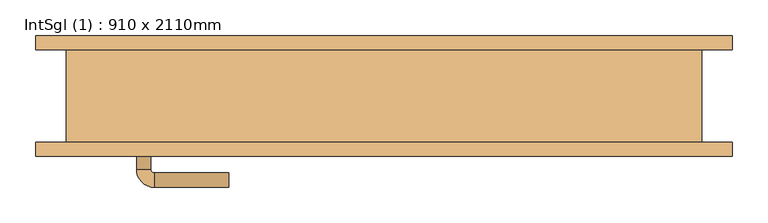
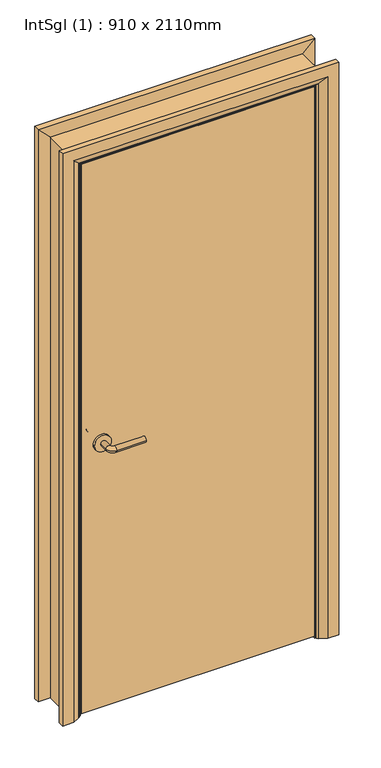
"""IFC4 building model written with IfcOpenShell, lengths in millimetres: door geometry, IntSgl (1) : 910 x 2110mm."""

import ifcopenshell
import ifcopenshell.guid

model = None  # the IFC model being written
_history = None  # IfcOwnerHistory: only IFC2X3 demands one
_inside = {}  # id of a spatial element -> (the spatial element, [elements in it])
_under = {}  # id of a project, library or spatial element -> (it, [spatial elements below it])
_declared = {}  # id of a project -> (the project, [libraries it declares])
_typed = {}  # id of a type object -> (the type object, [elements of that type])
_made_of = {}  # id of a material, layer set ... -> (it, [elements and type objects made of it])


def new_model(schema):
    """Start an empty IFC model of exactly this schema.

    Asked for "IFC4X3", IfcOpenShell would pick the latest addendum, in which some entities
    have other attributes; the version numbers below select the first issue.
    IFC2X3 requires an IfcOwnerHistory on every rooted entity: one is made here for all.
    """
    global model, _history
    if schema == "IFC4X3":
        model = ifcopenshell.file(schema_version=(4, 3, 0, 0))
    else:
        model = ifcopenshell.file(schema=schema)
    _inside.clear()
    _under.clear()
    _declared.clear()
    _typed.clear()
    _made_of.clear()
    _history = None
    if model.schema == "IFC2X3":
        org = make("IfcOrganization", Name="unknown")
        user = make(
            "IfcPersonAndOrganization",
            ThePerson=make("IfcPerson", FamilyName="unknown"),
            TheOrganization=org,
        )
        app = make(
            "IfcApplication",
            ApplicationDeveloper=org,
            Version="unknown",
            ApplicationFullName="unknown",
            ApplicationIdentifier="unknown",
        )
        _history = make(
            "IfcOwnerHistory",
            OwningUser=user,
            OwningApplication=app,
            ChangeAction="ADDED",
            CreationDate=0,
        )
    return model


def make(cls, **values):
    """One entity of the class cls with the attributes given. An attribute that is None is left unset."""
    return model.create_entity(
        cls, **{name: value for name, value in values.items() if value is not None}
    )


def rooted(cls, **values):
    """An entity with a GlobalId (a new one), such as an element, a storey or a relation."""
    return make(cls, GlobalId=ifcopenshell.guid.new(), OwnerHistory=_history, **values)


def si_unit(unit_type, name, prefix=None):
    """IfcSIUnit, for example si_unit("LENGTHUNIT", "METRE", prefix="MILLI")."""
    return make("IfcSIUnit", UnitType=unit_type, Prefix=prefix, Name=name)


def assignment(units):
    """IfcUnitAssignment: the units of a project."""
    return None if units is None else make("IfcUnitAssignment", Units=units)


def point(xyz):
    """IfcCartesianPoint."""
    return None if xyz is None else make("IfcCartesianPoint", Coordinates=xyz)


def direction(xyz):
    """IfcDirection."""
    return None if xyz is None else make("IfcDirection", DirectionRatios=xyz)


def frame(location, z_axis=None, x_axis=None):
    """IfcAxis2Placement3D, a coordinate frame: its origin and axes. An axis left out is left unset."""
    return make(
        "IfcAxis2Placement3D",
        Location=point(location),
        Axis=direction(z_axis),
        RefDirection=direction(x_axis),
    )


def frame_2d(location, x_axis=None):
    """IfcAxis2Placement2D, a coordinate frame in the plane: its origin and x axis."""
    return make(
        "IfcAxis2Placement2D", Location=point(location), RefDirection=direction(x_axis)
    )


def origin():
    """The frame at (0, 0, 0) with its axes left unset."""
    return frame((0.0, 0.0, 0.0))


def place(relative_to, where):
    """IfcLocalPlacement: puts the frame where relative to a parent placement (None: the world)."""
    return make(
        "IfcLocalPlacement", PlacementRelTo=relative_to, RelativePlacement=where
    )


def context(
    kind, dimensions, precision=None, world=None, true_north=None, identifier=None
):
    """IfcGeometricRepresentationContext, for example the 3D "Model" context."""
    return make(
        "IfcGeometricRepresentationContext",
        ContextIdentifier=identifier,
        ContextType=kind,
        CoordinateSpaceDimension=dimensions,
        Precision=precision,
        WorldCoordinateSystem=world,
        TrueNorth=true_north,
    )


def project(units=None, contexts=None):
    """IfcProject with its units and contexts."""
    return rooted(
        "IfcProject",
        Name="project",
        RepresentationContexts=contexts,
        UnitsInContext=assignment(units),
    )


def spatial(cls, under=None, at=None, **own):
    """A site, building, storey or space (cls), placed at a placement, below another one or the project."""
    s = rooted(cls, ObjectPlacement=at, **own)
    if under is not None:
        _under.setdefault(under.id(), (under, []))[1].append(s)
    return s


def polyline(points):
    """IfcPolyline through the points."""
    return make("IfcPolyline", Points=[point(p) for p in points])


def circle_curve(where, radius):
    """IfcCircle in the frame where."""
    return make("IfcCircle", Position=where, Radius=radius)


def ellipse_curve(where, semi_axis1, semi_axis2):
    """IfcEllipse in the frame where."""
    return make(
        "IfcEllipse", Position=where, SemiAxis1=semi_axis1, SemiAxis2=semi_axis2
    )


def trimmed(basis, trim1, trim2, sense, master):
    """IfcTrimmedCurve: the piece of a basis curve between two trims."""
    return make(
        "IfcTrimmedCurve",
        BasisCurve=basis,
        Trim1=trim1,
        Trim2=trim2,
        SenseAgreement=sense,
        MasterRepresentation=master,
    )


def segment(curve, same_sense, transition):
    """IfcCompositeCurveSegment."""
    return make(
        "IfcCompositeCurveSegment",
        Transition=transition,
        SameSense=same_sense,
        ParentCurve=curve,
    )


def composite_curve(segments, self_intersect=None):
    """IfcCompositeCurve: segments joined end to end."""
    return make("IfcCompositeCurve", Segments=segments, SelfIntersect=self_intersect)


def outline(outer, holes=None, kind="AREA"):
    """IfcArbitraryClosedProfileDef: a profile drawn as a closed curve; with holes, ...WithVoids."""
    if holes is None:
        return make("IfcArbitraryClosedProfileDef", ProfileType=kind, OuterCurve=outer)
    return make(
        "IfcArbitraryProfileDefWithVoids",
        ProfileType=kind,
        OuterCurve=outer,
        InnerCurves=holes,
    )


def extrude(swept, where, along, depth):
    """IfcExtrudedAreaSolid: the profile swept, set in the frame where, extruded along a direction by depth."""
    return make(
        "IfcExtrudedAreaSolid",
        SweptArea=swept,
        Position=where,
        ExtrudedDirection=direction(along),
        Depth=depth,
    )


def faces_of(points, faces, orient=None, outer=None):
    """IfcFace entities. A face is a list of loops; a loop is a list of indices into points, from 0.

    orient and outer hold one flag for each loop. By default every Orientation is true, the
    first loop of a face is its IfcFaceOuterBound and the others are IfcFaceBound.
    """
    made = []
    for i, loops in enumerate(faces):
        bounds = []
        for j, loop in enumerate(loops):
            is_outer = j == 0 if outer is None else outer[i][j]
            bounds.append(
                make(
                    "IfcFaceOuterBound" if is_outer else "IfcFaceBound",
                    Bound=make("IfcPolyLoop", Polygon=[points[k] for k in loop]),
                    Orientation=True if orient is None else orient[i][j],
                )
            )
        made.append(make("IfcFace", Bounds=bounds))
    return made


def faceted_brep(points, faces, orient=None, outer=None, voids=None):
    """IfcFacetedBrep: a solid bounded by flat faces; with voids (closed shells), ...WithVoids."""
    shared = [point(p) for p in points]
    hull = make("IfcClosedShell", CfsFaces=faces_of(shared, faces, orient, outer))
    if voids is None:
        return make("IfcFacetedBrep", Outer=hull)
    return make(
        "IfcFacetedBrepWithVoids",
        Outer=hull,
        Voids=[
            make(cls, CfsFaces=faces_of(shared, fs, o, b)) for cls, fs, o, b in voids
        ],
    )


def shape(context_of_items, identifier, shape_type, items):
    """IfcShapeRepresentation: the items that make up one representation, for example the "Body"."""
    return make(
        "IfcShapeRepresentation",
        ContextOfItems=context_of_items,
        RepresentationIdentifier=identifier,
        RepresentationType=shape_type,
        Items=items,
    )


def source(mapping_origin, context_of_items, identifier, shape_type, items):
    """IfcRepresentationMap: a shape defined once, which mapped items show again and again."""
    return make(
        "IfcRepresentationMap",
        MappingOrigin=mapping_origin,
        MappedRepresentation=shape(context_of_items, identifier, shape_type, items),
    )


def transform(
    local_origin,
    x_axis=None,
    y_axis=None,
    z_axis=None,
    scale=None,
    scale2=None,
    scale3=None,
    uniform=True,
):
    """IfcCartesianTransformationOperator3D, or its non-uniform kind. x_axis, y_axis, z_axis: its Axis1, 2, 3."""
    if uniform:
        return make(
            "IfcCartesianTransformationOperator3D",
            Axis1=direction(x_axis),
            Axis2=direction(y_axis),
            LocalOrigin=point(local_origin),
            Scale=scale,
            Axis3=direction(z_axis),
        )
    return make(
        "IfcCartesianTransformationOperator3DnonUniform",
        Axis1=direction(x_axis),
        Axis2=direction(y_axis),
        LocalOrigin=point(local_origin),
        Scale=scale,
        Axis3=direction(z_axis),
        Scale2=scale2,
        Scale3=scale3,
    )


def mapped(mapping_source, mapping_target):
    """IfcMappedItem: shows the shape of a source again, moved by a transform."""
    return make(
        "IfcMappedItem", MappingSource=mapping_source, MappingTarget=mapping_target
    )


def made_of(thing, what):
    """Note that an element or type object is made of a material, layer set ...; save() writes the relation."""
    if what is not None:
        _made_of.setdefault(what.id(), (what, []))[1].append(thing)
    return thing


def element(
    cls,
    number,
    at=None,
    inside=None,
    cuts=None,
    type_object=None,
    material=None,
    context=None,
    identifier="Body",
    shape_type=None,
    held_by="IfcProductDefinitionShape",
    body=None,
    shapes=None,
    **own,
):
    """One element of the class cls, such as IfcWall. Its Tag is "e" and its number.

    at: its placement. inside: the storey or other place that contains it. cuts: it is an
    opening in that element (IfcRelVoidsElement). A single representation is given by context,
    identifier, shape_type and body (its items); several are given by shapes. held_by: the class
    of the entity that holds the representations. save() writes the other relations.
    """
    e = rooted(cls, Tag="e%d" % number, ObjectPlacement=at, **own)
    if body is not None:
        shapes = [shape(context, identifier, shape_type, body)]
    if shapes is not None:
        e.Representation = make(held_by, Representations=shapes)
    if inside is not None:
        _inside.setdefault(inside.id(), (inside, []))[1].append(e)
    if cuts is not None:
        rooted(
            "IfcRelVoidsElement", RelatingBuildingElement=cuts, RelatedOpeningElement=e
        )
    if type_object is not None:
        _typed.setdefault(type_object.id(), (type_object, []))[1].append(e)
    return made_of(e, material)


def aggregate(whole, parts):
    """IfcRelAggregates: a whole, such as a stair, and the parts it consists of."""
    return rooted("IfcRelAggregates", RelatingObject=whole, RelatedObjects=parts)


def save(model, path):
    """Write the relations noted so far, then the file.

    IfcRelAggregates (storeys below a building ...), IfcRelContainedInSpatialStructure (elements
    in a storey), IfcRelDefinesByType, IfcRelAssociatesMaterial and IfcRelDeclares: one each for
    every whole, place, type object, material and project.
    """
    for whole, parts in _under.values():
        aggregate(whole, parts)
    for where, things in _inside.values():
        rooted(
            "IfcRelContainedInSpatialStructure",
            RelatedElements=things,
            RelatingStructure=where,
        )
    for kind, things in _typed.values():
        rooted("IfcRelDefinesByType", RelatedObjects=things, RelatingType=kind)
    for what, things in _made_of.values():
        rooted("IfcRelAssociatesMaterial", RelatedObjects=things, RelatingMaterial=what)
    for by, libraries in _declared.values():
        rooted("IfcRelDeclares", RelatingContext=by, RelatedDefinitions=libraries)
    model.write(path)


def plane_surface(at):
    """IfcPlane: the flat surface through the origin of the frame at, square to its z axis."""
    return make("IfcPlane", Position=at)


def cylinder_surface(at, radius):
    """IfcCylindricalSurface: all points at the distance radius from the z axis of the frame at."""
    return make("IfcCylindricalSurface", Position=at, Radius=radius)


def revolved_surface(curve, axis_point, axis_direction):
    """IfcSurfaceOfRevolution: the curve turned about the line through axis_point along axis_direction."""
    return make(
        "IfcSurfaceOfRevolution",
        SweptCurve=make("IfcArbitraryOpenProfileDef", ProfileType="CURVE", Curve=curve),
        AxisPosition=make("IfcAxis1Placement", Location=point(axis_point), Axis=direction(axis_direction)),
    )


def advanced_brep(points, edges, surfaces, faces):
    """IfcAdvancedBrep: a solid bounded by faces that lie on surfaces and meet in shared edges.

    An edge is (start, end): straight between two places in points (the first is 0);
    or (start, end, curve); or (start, end, curve, False) where it runs against its curve.
    A face is (place in surfaces, loops), or (place, loops, False) where it looks against
    its surface's normal. A loop lists edges by number (the first is 1), with a minus sign
    where the edge is run from its end to its start. The first loop is the outer one.
    """
    corners = [point(p) for p in points]
    vertices = [make("IfcVertexPoint", VertexGeometry=c) for c in corners]
    made = []
    for start, end, *more in edges:
        made.append(
            make(
                "IfcEdgeCurve",
                EdgeStart=vertices[start],
                EdgeEnd=vertices[end],
                EdgeGeometry=more[0] if more else make("IfcPolyline", Points=[corners[start], corners[end]]),
                SameSense=more[1] if len(more) > 1 else True,
            )
        )
    hull = []
    for where, loops, *sense in faces:
        bounds = []
        for j, loop in enumerate(loops):
            ring = [make("IfcOrientedEdge", EdgeElement=made[abs(k) - 1], Orientation=k > 0) for k in loop]
            bounds.append(
                make(
                    "IfcFaceOuterBound" if j == 0 else "IfcFaceBound",
                    Bound=make("IfcEdgeLoop", EdgeList=ring),
                    Orientation=True,
                )
            )
        hull.append(make("IfcAdvancedFace", Bounds=bounds, FaceSurface=surfaces[where], SameSense=sense[0] if sense else True))
    return make("IfcAdvancedBrep", Outer=make("IfcClosedShell", CfsFaces=hull))


def intsgl_1_910_x_2110mm_ad2476ae(model_context):
    return source(origin(), model_context, "Body", "SolidModel", [
        advanced_brep(
        [(-348.0, -19.0, 1000.0), (-328.0, -19.0, 1000.0), (-348.0, 11.0, 1000.0), (-328.0, 11.0, 1000.0), (-323.0, 16.0, 1000.0), (-323.0, 36.0, 1000.0), (-218.0, 36.0, 1000.0), (-218.0, 16.0, 1000.0)],
        [
            (0, 1, circle_curve(frame((-338.0, -19.0, 1000.0), z_axis=(0.0, -1.0, 0.0), x_axis=(1.0, 0.0, 0.0)), 10.0)),
            (1, 0, circle_curve(frame((-338.0, -19.0, 1000.0), z_axis=(0.0, -1.0, 0.0), x_axis=(1.0, 0.0, 0.0)), 10.0)),
            (0, 2),
            (2, 3, circle_curve(frame((-338.0, 11.0, 1000.0), z_axis=(0.0, -1.0, 0.0), x_axis=(1.0, 0.0, 0.0)), 10.0)),
            (3, 1),
            (3, 2, circle_curve(frame((-338.0, 11.0, 1000.0), z_axis=(0.0, -1.0, 0.0), x_axis=(1.0, 0.0, 0.0)), 10.0)),
            (4, 3, circle_curve(frame((-323.0, 11.0, 1000.0), z_axis=(0.0, 0.0, 1.0), x_axis=(-1.0, 0.0, 0.0)), 5.0)),
            (2, 5, circle_curve(frame((-323.0, 11.0, 1000.0), z_axis=(0.0, 0.0, -1.0), x_axis=(-1.0, 0.0, 0.0)), 25.0)),
            (5, 4, circle_curve(frame((-323.0, 26.0, 1000.0), z_axis=(-1.0, 0.0, 0.0), x_axis=(0.0, -1.0, 0.0)), 10.0)),
            (4, 5, circle_curve(frame((-323.0, 26.0, 1000.0), z_axis=(-1.0, 0.0, 0.0), x_axis=(0.0, -1.0, 0.0)), 10.0)),
            (6, 7, circle_curve(frame((-218.0, 26.0, 1000.0), z_axis=(1.0, 0.0, 0.0), x_axis=(0.0, -1.0, 0.0)), 10.0)),
            (7, 6, circle_curve(frame((-218.0, 26.0, 1000.0), z_axis=(1.0, 0.0, 0.0), x_axis=(0.0, -1.0, 0.0)), 10.0)),
            (5, 6),
            (7, 4),
        ],
        [
            plane_surface(frame((-338.0, -19.0, 1000.0), z_axis=(0.0, -1.0, 0.0), x_axis=(0.0, 0.0, 1.0))),
            cylinder_surface(frame((-338.0, -19.0, 1000.0), z_axis=(0.0, -1.0, 0.0), x_axis=(1.0, 0.0, 0.0)), 10.0),
            revolved_surface(trimmed(ellipse_curve(frame((-338.0, 11.0, 1000.0), z_axis=(0.0, -1.0, 0.0), x_axis=(1.0, 0.0, 0.0)), 10.0, 10.0), [point((-348.0, 11.0, 1000.0))], [point((-328.0, 11.0, 1000.0))], True, "CARTESIAN"), (-323.0, 11.0, 1000.0), (0.0, 0.0, -1.0)),
            revolved_surface(trimmed(ellipse_curve(frame((-338.0, 11.0, 1000.0), z_axis=(0.0, -1.0, 0.0), x_axis=(1.0, 0.0, 0.0)), 10.0, 10.0), [point((-328.0, 11.0, 1000.0))], [point((-348.0, 11.0, 1000.0))], True, "CARTESIAN"), (-323.0, 11.0, 1000.0), (0.0, 0.0, -1.0)),
            plane_surface(frame((-218.0, 26.0, 1000.0), z_axis=(1.0, 0.0, 0.0), x_axis=(0.0, 0.0, 1.0))),
            cylinder_surface(frame((-323.0, 26.0, 1000.0), z_axis=(-1.0, 0.0, 0.0), x_axis=(0.0, -1.0, 0.0)), 10.0),
        ],
        [
            (0, [[1, 2]]),
            (1, [[-1, 3, 4, 5]]),
            (1, [[-2, -5, 6, -3]]),
            (2, [[7, -4, 8, 9]]),
            (3, [[-8, -6, -7, 10]]),
            (4, [[11, 12]]),
            (5, [[-9, 13, -12, 14]]),
            (5, [[-10, -14, -11, -13]]),
        ],
    ),
        extrude(outline(composite_curve([segment(trimmed(circle_curve(frame_2d((1000.0, -340.5)), 30.0), [point((1000.0, -370.5))], [point((1000.0, -310.5))], False, "CARTESIAN"), True, "CONTINUOUS"), segment(trimmed(circle_curve(frame_2d((1000.0, -340.5)), 30.0), [point((1000.0, -310.5))], [point((1000.0, -370.5))], False, "CARTESIAN"), True, "CONTINUOUS")], self_intersect=False)), frame((0.0, -27.0, 0.0), z_axis=(0.0, 1.0, 0.0), x_axis=(0.0, 0.0, 1.0)), (0.0, 0.0, 1.0), 8.0),
        advanced_brep(
        [(-348.0, -73.0, 1000.0), (-328.0, -73.0, 1000.0), (-328.0, -103.0, 1000.0), (-348.0, -103.0, 1000.0), (-323.0, -108.0, 1000.0), (-323.0, -128.0, 1000.0), (-218.0, -128.0, 1000.0), (-218.0, -108.0, 1000.0)],
        [
            (0, 1, circle_curve(frame((-338.0, -73.0, 1000.0), z_axis=(0.0, 1.0, 0.0), x_axis=(1.0, 0.0, 0.0)), 10.0)),
            (1, 0, circle_curve(frame((-338.0, -73.0, 1000.0), z_axis=(0.0, 1.0, 0.0), x_axis=(1.0, 0.0, 0.0)), 10.0)),
            (1, 2),
            (2, 3, circle_curve(frame((-338.0, -103.0, 1000.0), z_axis=(0.0, 1.0, 0.0), x_axis=(1.0, 0.0, 0.0)), 10.0)),
            (3, 0),
            (3, 2, circle_curve(frame((-338.0, -103.0, 1000.0), z_axis=(0.0, 1.0, 0.0), x_axis=(1.0, 0.0, 0.0)), 10.0)),
            (4, 5, circle_curve(frame((-323.0, -118.0, 1000.0), z_axis=(-1.0, 0.0, 0.0), x_axis=(0.0, 1.0, 0.0)), 10.0)),
            (5, 3, circle_curve(frame((-323.0, -103.0, 1000.0), z_axis=(0.0, 0.0, -1.0), x_axis=(-1.0, 0.0, 0.0)), 25.0)),
            (2, 4, circle_curve(frame((-323.0, -103.0, 1000.0), z_axis=(0.0, 0.0, 1.0), x_axis=(-1.0, 0.0, 0.0)), 5.0)),
            (5, 4, circle_curve(frame((-323.0, -118.0, 1000.0), z_axis=(-1.0, 0.0, 0.0), x_axis=(0.0, 1.0, 0.0)), 10.0)),
            (6, 7, circle_curve(frame((-218.0, -118.0, 1000.0), z_axis=(1.0, 0.0, 0.0), x_axis=(0.0, 1.0, 0.0)), 10.0)),
            (7, 6, circle_curve(frame((-218.0, -118.0, 1000.0), z_axis=(1.0, 0.0, 0.0), x_axis=(0.0, 1.0, 0.0)), 10.0)),
            (4, 7),
            (6, 5),
        ],
        [
            plane_surface(frame((-338.0, -73.0, 1000.0), z_axis=(0.0, 1.0, 0.0), x_axis=(0.0, 0.0, 1.0))),
            cylinder_surface(frame((-338.0, -73.0, 1000.0), z_axis=(0.0, 1.0, 0.0), x_axis=(1.0, 0.0, 0.0)), 10.0),
            revolved_surface(trimmed(ellipse_curve(frame((-338.0, -103.0, 1000.0), z_axis=(0.0, -1.0, 0.0), x_axis=(1.0, 0.0, 0.0)), 10.0, 10.0), [point((-348.0, -103.0, 1000.0))], [point((-328.0, -103.0, 1000.0))], True, "CARTESIAN"), (-323.0, -103.0, 1000.0), (0.0, 0.0, -1.0)),
            revolved_surface(trimmed(ellipse_curve(frame((-338.0, -103.0, 1000.0), z_axis=(0.0, -1.0, 0.0), x_axis=(1.0, 0.0, 0.0)), 10.0, 10.0), [point((-328.0, -103.0, 1000.0))], [point((-348.0, -103.0, 1000.0))], True, "CARTESIAN"), (-323.0, -103.0, 1000.0), (0.0, 0.0, -1.0)),
            plane_surface(frame((-218.0, -118.0, 1000.0), z_axis=(1.0, 0.0, 0.0), x_axis=(0.0, 0.0, 1.0))),
            cylinder_surface(frame((-323.0, -118.0, 1000.0), z_axis=(-1.0, 0.0, 0.0), x_axis=(0.0, 1.0, 0.0)), 10.0),
        ],
        [
            (0, [[1, 2]]),
            (1, [[3, 4, 5, -2]]),
            (1, [[-5, 6, -3, -1]]),
            (2, [[7, 8, -4, 9]]),
            (3, [[10, -9, -6, -8]]),
            (4, [[11, 12]]),
            (5, [[13, -11, 14, -7]]),
            (5, [[-14, -12, -13, -10]]),
        ],
    ),
        extrude(outline(composite_curve([segment(trimmed(circle_curve(frame_2d((1000.0, -340.5)), 30.0), [point((1000.0, -370.5))], [point((1000.0, -310.5))], False, "CARTESIAN"), True, "CONTINUOUS"), segment(trimmed(circle_curve(frame_2d((1000.0, -340.5)), 30.0), [point((1000.0, -310.5))], [point((1000.0, -370.5))], False, "CARTESIAN"), True, "CONTINUOUS")], self_intersect=False)), frame((0.0, -73.0, 0.0), z_axis=(0.0, 1.0, 0.0), x_axis=(0.0, 0.0, 1.0)), (0.0, 0.0, 1.0), 8.0),
        extrude(outline(polyline([(413.0, -27.0), (413.0, -65.0), (-413.0, -65.0), (-413.0, -27.0), (413.0, -27.0)])), frame((0.0, 0.0, 8.0), z_axis=(0.0, 0.0, 1.0), x_axis=(1.0, 0.0, 0.0)), (0.0, 0.0, 1.0), 2060.0),
        advanced_brep(
        [(490.0, -85.0, 0.0), (450.0, -85.0, 0.0), (424.0, -71.0, 0.0), (420.0, -65.0, 0.0), (490.0, -65.0, 0.0), (490.0, -65.0, 2145.0), (490.0, -85.0, 2145.0), (420.0, -65.0, 2075.0), (-420.0, -65.0, 2075.0), (-420.0, -65.0, 0.0), (-490.0, -65.0, 0.0), (-490.0, -65.0, 2145.0), (424.0, -71.0, 2079.0), (450.0, -85.0, 2105.0), (-490.0, -85.0, 2145.0), (-490.0, -85.0, 0.0), (-450.0, -85.0, 0.0), (-450.0, -85.0, 2105.0), (-424.0, -71.0, 2079.0), (-424.0, -71.0, 0.0)],
        [
            (0, 1),
            (1, 2),
            (2, 3, circle_curve(frame((428.0, -64.0, 0.0), z_axis=(0.0, 0.0, -1.0), x_axis=(1.0, 0.0, 0.0)), 8.0622577)),
            (3, 4),
            (4, 0),
            (4, 5),
            (5, 6),
            (6, 0),
            (3, 7),
            (7, 8),
            (8, 9),
            (9, 10),
            (10, 11),
            (11, 5),
            (2, 12),
            (12, 7, ellipse_curve(frame((428.0, -64.0, 2083.0), z_axis=(0.7071067811865475, 0.0, -0.7071067811865475), x_axis=(-0.7071067811865474, 0.0, -0.7071067811865476)), 11.4017543, 8.0622577)),
            (1, 13),
            (13, 12),
            (6, 14),
            (14, 15),
            (15, 16),
            (16, 17),
            (17, 13),
            (11, 14),
            (12, 18),
            (18, 8, ellipse_curve(frame((-428.0, -64.0, 2083.0), z_axis=(0.7071067811865475, 0.0, 0.7071067811865475), x_axis=(0.7071067811865476, 0.0, -0.7071067811865474)), 11.4017543, 8.0622577)),
            (17, 18),
            (15, 10),
            (9, 19, circle_curve(frame((-428.0, -64.0, 0.0), z_axis=(0.0, 0.0, -1.0), x_axis=(-1.0, 0.0, 0.0)), 8.0622577)),
            (19, 16),
            (18, 19),
        ],
        [
            plane_surface(frame((420.0, -65.0, 0.0), z_axis=(0.0, 0.0, -1.0), x_axis=(0.0, 1.0, 0.0))),
            plane_surface(frame((490.0, -85.0, 0.0), z_axis=(1.0, 0.0, 0.0), x_axis=(0.0, 0.0, 1.0))),
            plane_surface(frame((490.0, -65.0, 0.0), z_axis=(0.0, 1.0, 0.0), x_axis=(0.0, 0.0, 1.0))),
            cylinder_surface(frame((428.0, -64.0, 0.0), z_axis=(0.0, 0.0, -1.0), x_axis=(1.0, 0.0, 0.0)), 8.0622577),
            plane_surface(frame((424.0, -71.0, 0.0), z_axis=(-0.4740998230350126, -0.880471099922178, 0.0), x_axis=(0.0, 0.0, 1.0))),
            plane_surface(frame((450.0, -85.0, 0.0), z_axis=(0.0, -1.0, 0.0), x_axis=(0.0, 0.0, 1.0))),
            plane_surface(frame((490.0, -85.0, 2145.0), z_axis=(0.0, 0.0, 1.0), x_axis=(-1.0, 0.0, 0.0))),
            cylinder_surface(frame((420.0, -64.0, 2083.0), z_axis=(1.0, 0.0, 0.0), x_axis=(0.0, 0.0, 1.0)), 8.0622577),
            plane_surface(frame((424.0, -71.0, 2079.0), z_axis=(0.0, -0.8804710999221764, -0.4740998230350154), x_axis=(-1.0, 0.0, 0.0))),
            plane_surface(frame((-420.0, -65.0, 0.0), z_axis=(0.0, 0.0, -1.0), x_axis=(0.0, 1.0, 0.0))),
            plane_surface(frame((-490.0, -85.0, 2145.0), z_axis=(-1.0, 0.0, 0.0), x_axis=(0.0, 0.0, -1.0))),
            cylinder_surface(frame((-428.0, -64.0, 2075.0), z_axis=(0.0, 0.0, 1.0), x_axis=(-1.0, 0.0, 0.0)), 8.0622577),
            plane_surface(frame((-424.0, -71.0, 2079.0), z_axis=(0.47409982303501824, -0.8804710999221749, 0.0), x_axis=(0.0, 0.0, -1.0))),
        ],
        [
            (0, [[1, 2, 3, 4, 5]]),
            (1, [[6, 7, 8, -5]]),
            (2, [[9, 10, 11, 12, 13, 14, -6, -4]]),
            (3, [[15, 16, -9, -3]]),
            (4, [[17, 18, -15, -2]]),
            (5, [[-8, 19, 20, 21, 22, 23, -17, -1]]),
            (6, [[-14, 24, -19, -7]]),
            (7, [[25, 26, -10, -16]]),
            (8, [[-23, 27, -25, -18]]),
            (9, [[28, -12, 29, 30, -21]]),
            (10, [[-13, -28, -20, -24]]),
            (11, [[31, -29, -11, -26]]),
            (12, [[-22, -30, -31, -27]]),
        ],
    ),
        extrude(outline(polyline([(0.0, -396.0), (2051.0, -396.0), (2051.0, 396.0), (0.0, 396.0), (0.0, 415.0), (2070.0, 415.0), (2070.0, -415.0), (0.0, -415.0), (0.0, -396.0)])), frame((0.0, -25.0, 0.0), z_axis=(0.0, 1.0, 0.0), x_axis=(0.0, 0.0, 1.0)), (0.0, 0.0, 1.0), 32.0),
        advanced_brep(
        [(-490.0, 85.0, 0.0), (-450.0, 85.0, 0.0), (-424.0, 71.0, 0.0), (-420.0, 65.0, 0.0), (-490.0, 65.0, 0.0), (-490.0, 65.0, 2145.0), (-490.0, 85.0, 2145.0), (-420.0, 65.0, 2075.0), (-424.0, 71.0, 2079.0), (-450.0, 85.0, 2105.0), (490.0, 65.0, 2145.0), (490.0, 85.0, 2145.0), (420.0, 65.0, 2075.0), (424.0, 71.0, 2079.0), (450.0, 85.0, 2105.0), (490.0, 85.0, 0.0), (490.0, 65.0, 0.0), (420.0, 65.0, 0.0), (424.0, 71.0, 0.0), (450.0, 85.0, 0.0)],
        [
            (0, 1),
            (1, 2),
            (2, 3, circle_curve(frame((-428.0, 64.0, 0.0), z_axis=(0.0, 0.0, -1.0), x_axis=(-1.0, 0.0, 0.0)), 8.0622577)),
            (3, 4),
            (4, 0),
            (4, 5),
            (5, 6),
            (6, 0),
            (3, 7),
            (7, 5),
            (2, 8),
            (8, 7, ellipse_curve(frame((-428.0, 64.0, 2083.0), z_axis=(-0.7071067811865475, 0.0, -0.7071067811865475), x_axis=(0.7071067811865474, 0.0, -0.7071067811865476)), 11.4017543, 8.0622577)),
            (1, 9),
            (9, 8),
            (6, 9),
            (5, 10),
            (10, 11),
            (11, 6),
            (7, 12),
            (12, 10),
            (8, 13),
            (13, 12, ellipse_curve(frame((428.0, 64.0, 2083.0), z_axis=(-0.7071067811865475, 0.0, 0.7071067811865475), x_axis=(-0.7071067811865476, 0.0, -0.7071067811865474)), 11.4017543, 8.0622577)),
            (9, 14),
            (14, 13),
            (11, 14),
            (15, 16),
            (16, 17),
            (17, 18, circle_curve(frame((428.0, 64.0, 0.0), z_axis=(0.0, 0.0, -1.0), x_axis=(1.0, 0.0, 0.0)), 8.0622577)),
            (18, 19),
            (19, 15),
            (10, 16),
            (15, 11),
            (12, 17),
            (13, 18),
            (14, 19),
        ],
        [
            plane_surface(frame((-420.0, 137.8010989, 0.0), z_axis=(0.0, 0.0, -1.0), x_axis=(1.0, 0.0, 0.0))),
            plane_surface(frame((-490.0, 85.0, 0.0), z_axis=(-1.0, 0.0, 0.0), x_axis=(0.0, 0.0, 1.0))),
            plane_surface(frame((-490.0, 65.0, 0.0), z_axis=(0.0, -1.0, 0.0), x_axis=(0.0, 0.0, 1.0))),
            cylinder_surface(frame((-428.0, 64.0, 0.0), z_axis=(0.0, 0.0, -1.0), x_axis=(-1.0, 0.0, 0.0)), 8.0622577),
            plane_surface(frame((-424.0, 71.0, 0.0), z_axis=(0.4740998230350183, 0.8804710999221749, 0.0), x_axis=(0.0, 0.0, 1.0))),
            plane_surface(frame((-450.0, 85.0, 0.0), z_axis=(0.0, 1.0, 0.0), x_axis=(0.0, 0.0, 1.0))),
            plane_surface(frame((-490.0, 85.0, 2145.0), z_axis=(0.0, 0.0, 1.0), x_axis=(1.0, 0.0, 0.0))),
            plane_surface(frame((-490.0, 65.0, 2145.0), z_axis=(0.0, -1.0, 0.0), x_axis=(1.0, 0.0, 0.0))),
            cylinder_surface(frame((-420.0, 64.0, 2083.0), z_axis=(-1.0, 0.0, 0.0), x_axis=(0.0, 0.0, 1.0)), 8.0622577),
            plane_surface(frame((-424.0, 71.0, 2079.0), z_axis=(0.0, 0.8804710999221749, -0.4740998230350183), x_axis=(1.0, 0.0, 0.0))),
            plane_surface(frame((-450.0, 85.0, 2105.0), z_axis=(0.0, 1.0, 0.0), x_axis=(1.0, 0.0, 0.0))),
            plane_surface(frame((420.0, 137.8010989, 0.0), z_axis=(0.0, 0.0, -1.0), x_axis=(-1.0, 0.0, 0.0))),
            plane_surface(frame((490.0, 85.0, 2145.0), z_axis=(1.0, 0.0, 0.0), x_axis=(0.0, 0.0, -1.0))),
            plane_surface(frame((490.0, 65.0, 2145.0), z_axis=(0.0, -1.0, 0.0), x_axis=(0.0, 0.0, -1.0))),
            cylinder_surface(frame((428.0, 64.0, 2075.0), z_axis=(0.0, 0.0, 1.0), x_axis=(1.0, 0.0, 0.0)), 8.0622577),
            plane_surface(frame((424.0, 71.0, 2079.0), z_axis=(-0.4740998230350183, 0.8804710999221749, 0.0), x_axis=(0.0, 0.0, -1.0))),
            plane_surface(frame((450.0, 85.0, 2105.0), z_axis=(0.0, 1.0, 0.0), x_axis=(0.0, 0.0, -1.0))),
        ],
        [
            (0, [[1, 2, 3, 4, 5]]),
            (1, [[6, 7, 8, -5]]),
            (2, [[9, 10, -6, -4]]),
            (3, [[11, 12, -9, -3]]),
            (4, [[13, 14, -11, -2]]),
            (5, [[-8, 15, -13, -1]]),
            (6, [[16, 17, 18, -7]]),
            (7, [[19, 20, -16, -10]]),
            (8, [[21, 22, -19, -12]]),
            (9, [[23, 24, -21, -14]]),
            (10, [[-18, 25, -23, -15]]),
            (11, [[26, 27, 28, 29, 30]]),
            (12, [[31, -26, 32, -17]]),
            (13, [[33, -27, -31, -20]]),
            (14, [[34, -28, -33, -22]]),
            (15, [[35, -29, -34, -24]]),
            (16, [[-32, -30, -35, -25]]),
        ],
    ),
        faceted_brep([(-415.0, -65.0, 0.0), (-447.0, -65.0, 0.0), (-447.0, 65.0, 0.0), (-415.0, 65.0, 0.0), (-415.0, 65.0, 2070.0), (-415.0, -65.0, 2070.0), (-447.0, 65.0, 2102.0), (-447.0, -65.0, 2102.0), (415.0, 65.0, 2070.0), (415.0, -65.0, 2070.0), (447.0, 65.0, 2102.0), (447.0, -65.0, 2102.0), (415.0, -65.0, 0.0), (415.0, 65.0, 0.0), (447.0, 65.0, 0.0), (447.0, -65.0, 0.0)], [[[0, 1, 2, 3]], [[3, 4, 5, 0]], [[2, 6, 4, 3]], [[1, 7, 6, 2]], [[0, 5, 7, 1]], [[4, 8, 9, 5]], [[6, 10, 8, 4]], [[7, 11, 10, 6]], [[5, 9, 11, 7]], [[12, 13, 14, 15]], [[8, 13, 12, 9]], [[10, 14, 13, 8]], [[11, 15, 14, 10]], [[9, 12, 15, 11]]]),
    ])


if __name__ == "__main__":
    model = new_model("IFC4")
    model_context = context("Model", 3, world=origin())
    ifc_project = project(units=[si_unit("LENGTHUNIT", "METRE", prefix="MILLI")], contexts=[model_context])
    site = spatial("IfcSite", under=ifc_project)
    building = spatial("IfcBuilding", under=site)
    placement = place(None, origin())
    intsgl_1_910_x_2110mm_shape = intsgl_1_910_x_2110mm_ad2476ae(model_context)
    element("IfcDoor", 1, ObjectType="IntSgl (1) : 910 x 2110mm", at=placement, inside=building, context=model_context, shape_type="MappedRepresentation", body=[
        mapped(intsgl_1_910_x_2110mm_shape, transform((0.0, 0.0, 0.0), x_axis=(1.0, 0.0, 0.0), y_axis=(0.0, 1.0, 0.0), z_axis=(0.0, 0.0, 1.0))),
    ])
    save(model, "model.ifc")

# Revit data of these elements
# Project information
#   Project Status = "Project Status"
#   Client Name = "Revit Project"
#   Project Address = "Enter address here"
#   Project Name = "Two Storey Residence"
#   Project Number = "P.01"
# Type "IntSgl (1) : 910 x 2110mm"
#   Construction Type Id = "MDOOR"
#   Analytic Construction = "Metal"
#   Type Mark = "41"
#   Type Comments = "Internal Single"
#   Operation = "SingleSwingRight"
#   Manufacturer = "Revit"
#   Keynote = "L20"
#   Description = "Internal Single Door"
#   Visual Light Transmittance = 0
#   Solar Heat Gain Coefficient = 0
#   Heat Transfer Coefficient (U) = 3.7021 W/(m²·K)
#   UnderCut = 8 mm
#   Tolerance = 2 mm
#   Thickness = 38 mm
#   Structural Tolerance = 8 mm
#   StopDepth = 32 mm
#   Stop Thickness = 19 mm
#   Rough Width = 910 mm
#   Rough Height = 2110 mm
#   Height to Top Lock Rail = 1000 mm
#   Handle Z Distance = 1000 mm
#   Handle X Distance = 75 mm
#   Frame Thickness = 32 mm
#   Door Panel Width = 826 mm
#   Door Panel Thickness = 38 mm
#   Door Panel Offset = 0 mm
#   Height = 2110 mm
#   Width = 910 mm
#   Door Panel Height = 2060 mm
#   Architrave Setback = 5 mm
#   Function = 0
#   Vis - Ironmongery = yes
#   Material Ironmongery = Door - Handle
#   Material Frame = Door - Frame/Mullion (1)
#   Material Door = Door - Panel
#   Material Architrave = Door - Architrave
#   Wall Closure = (empty or 0)
# Element 1 (IfcDoor, "IntSgl (1) : 910 x 2110mm")
#   Materials on its faces: "Door - Architrave", "Door - Handle", "Door - Frame/Mullion (1)", "Door - Panel"
# Materials
#   "Door - Handle": class "Miscellaneous", colour RGB 0 0 0, transparency 0, Keynote = "P21"
#   "Door - Frame/Mullion (1)": class "Wood", colour RGB 212 179 113, transparency 0, Keynote = "L20", Cost = 0
#   "Door - Panel": class "Wood", colour RGB 210 159 95, transparency 0, Keynote = "L20"
#   "Door - Architrave": class "Wood", colour RGB 154 90 5, transparency 0, Keynote = "P20"
